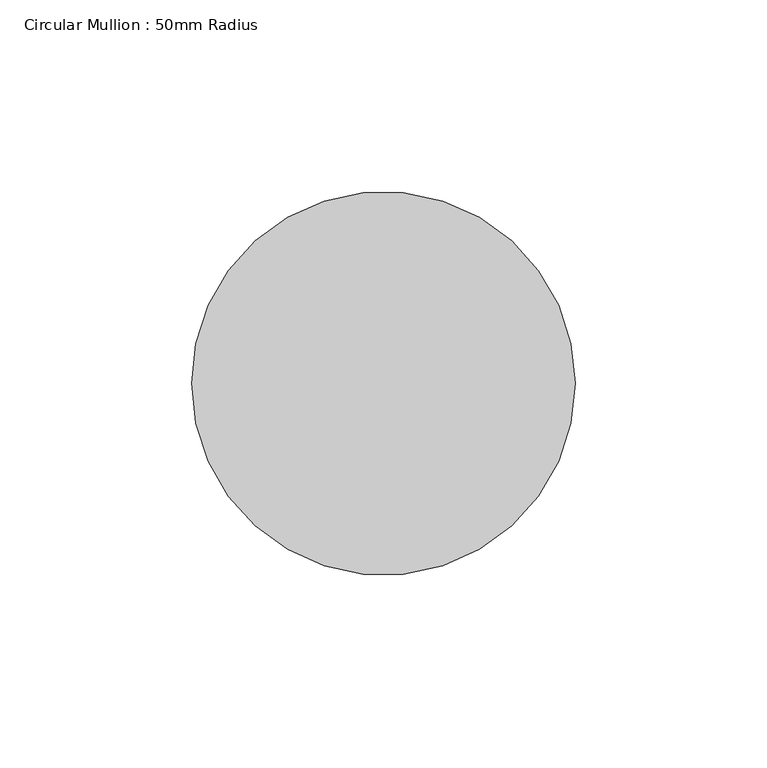
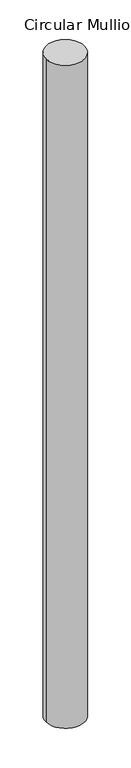
"""IFC4 building model written with IfcOpenShell, lengths in millimetres: member geometry, Circular Mullion : 50mm Radius."""

from ifc_helpers import new_model, si_unit, point, frame, origin, origin_2d, place, context, project, spatial, circle_curve, trimmed, segment, composite_curve, outline, extrude, source, transform, mapped, element, save


def circular_mullion_50mm_radius_1a05c7d5(model_context):
    return source(origin(), model_context, "Body", "SweptSolid", [
        extrude(outline(composite_curve([segment(trimmed(circle_curve(origin_2d(), 50.0), [point((50.0, 0.0))], [point((-50.0, 0.0))], False, "CARTESIAN"), True, "CONTINUOUS"), segment(trimmed(circle_curve(origin_2d(), 50.0), [point((-50.0, 0.0))], [point((50.0, 0.0))], False, "CARTESIAN"), True, "CONTINUOUS")], self_intersect=False)), frame((0.0, 0.0, -1803.5876195), z_axis=(0.0, 0.0, 1.0), x_axis=(1.0, 0.0, 0.0)), (0.0, 0.0, 1.0), 1803.5876195),
    ])


if __name__ == "__main__":
    model = new_model("IFC4")
    model_context = context("Model", 3, world=origin())
    ifc_project = project(units=[si_unit("LENGTHUNIT", "METRE", prefix="MILLI")], contexts=[model_context])
    site = spatial("IfcSite", under=ifc_project)
    building = spatial("IfcBuilding", under=site)
    placement = place(None, origin())
    circular_mullion_50mm_radius_shape = circular_mullion_50mm_radius_1a05c7d5(model_context)
    element("IfcMember", 1, ObjectType="Circular Mullion : 50mm Radius", at=placement, inside=building, context=model_context, shape_type="MappedRepresentation", body=[
        mapped(circular_mullion_50mm_radius_shape, transform((0.0, 0.0, 0.0), x_axis=(1.0, 0.0, 0.0), y_axis=(0.0, 1.0, 0.0), z_axis=(0.0, 0.0, 1.0))),
    ])
    save(model, "model.ifc")

# Revit data of these elements
# Type "Circular Mullion : 50mm Radius"
#   built-in parameter 1007350 = 0.164042 (stored number, unit not read)
# Element 1 (IfcMember, "Circular Mullion : 50mm Radius")
#   Materials on its faces: "Aluminium"
# Materials
#   "Aluminium": class "Metal", colour RGB 247 247 247, transparency 0, Description = "Aluminium 6061", Cost = 0
